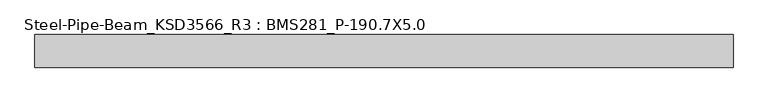
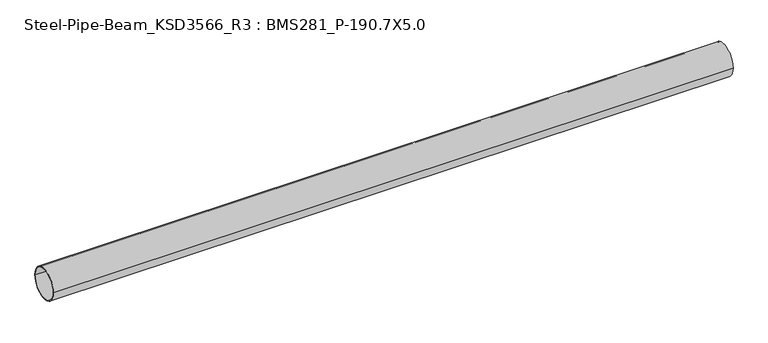
"""IFC4 building model written with IfcOpenShell, lengths in millimetres: member geometry, Steel-Pipe-Beam_KSD3566_R3 : BMS281_P-190.7X5.0."""

from ifc_helpers import new_model, si_unit, point, frame, origin, origin_2d, place, context, project, spatial, circle_curve, trimmed, segment, composite_curve, outline, extrude, source, transform, mapped, element, save


def steel_pipe_beam_ksd3566_r3_bms281_p_190_7x5_0_d858548f(model_context):
    return source(origin(), model_context, "Body", "SweptSolid", [
        extrude(outline(composite_curve([segment(trimmed(circle_curve(origin_2d(), 95.35), [point((-95.35, 0.0))], [point((95.35, 0.0))], False, "CARTESIAN"), True, "CONTINUOUS"), segment(trimmed(circle_curve(origin_2d(), 95.35), [point((95.35, 0.0))], [point((-95.35, 0.0))], False, "CARTESIAN"), True, "CONTINUOUS")], self_intersect=False), holes=[composite_curve([segment(trimmed(circle_curve(origin_2d(), 90.35), [point((90.35, 0.0))], [point((-90.35, 0.0))], True, "CARTESIAN"), True, "CONTINUOUS"), segment(trimmed(circle_curve(origin_2d(), 90.35), [point((-90.35, 0.0))], [point((90.35, 0.0))], True, "CARTESIAN"), True, "CONTINUOUS")], self_intersect=False)]), frame((-2028.8524281, 0.0, 0.0), z_axis=(1.0, 0.0, 0.0), x_axis=(0.0, 1.0, 0.0)), (0.0, 0.0, 1.0), 4074.9898367),
    ])


if __name__ == "__main__":
    model = new_model("IFC4")
    model_context = context("Model", 3, world=origin())
    ifc_project = project(units=[si_unit("LENGTHUNIT", "METRE", prefix="MILLI")], contexts=[model_context])
    site = spatial("IfcSite", under=ifc_project)
    building = spatial("IfcBuilding", under=site)
    placement = place(None, origin())
    steel_pipe_beam_ksd3566_r3_bms281_p_190_7x5_0_shape = steel_pipe_beam_ksd3566_r3_bms281_p_190_7x5_0_d858548f(model_context)
    element("IfcMember", 1, ObjectType="Steel-Pipe-Beam_KSD3566_R3 : BMS281_P-190.7X5.0", at=placement, inside=building, context=model_context, shape_type="MappedRepresentation", body=[
        mapped(steel_pipe_beam_ksd3566_r3_bms281_p_190_7x5_0_shape, transform((0.0, 0.0, 0.0), x_axis=(1.0, 0.0, 0.0), y_axis=(0.0, 1.0, 0.0), z_axis=(0.0, 0.0, 1.0))),
    ])
    save(model, "model.ifc")

# Revit data of these elements
# Type "Steel-Pipe-Beam_KSD3566_R3 : BMS281_P-190.7X5.0"
#   Keynote = "P-190.7X5.0"
#   SteelWeight = "Light"
#   t = 0.0050 m
#   Surface Area = 0.599102 m²/m
#   Section Area = 29.1697 cm²
#   Mass per Unit Length = 22.8982 kg/m
#   Length [instance default] = 1.5000 m
#   D = 0.1907 m
#   hec_material4 [instance default] = none
#   hec_material3 [instance default] = none
#   hec_material2 [instance default] = none
#   hec_material1 [instance default] = none
#   Structural Material [instance default] = Steel, 45-345
#   Assembly Code = ""
# Element 1 (IfcMember, "Steel-Pipe-Beam_KSD3566_R3 : BMS281_P-190.7X5.0")
#   Structural Material = none
# Materials
#   "Steel, 45-345": class "Metal", colour RGB 189 187 185, transparency 0, Description = "Steel 345 MPa", Cost = 0
